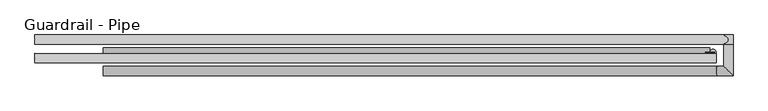
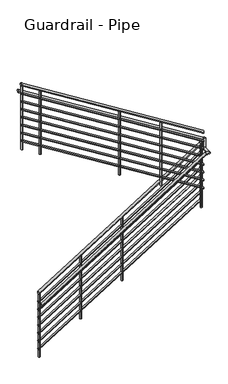
"""IFC4 building model written with IfcOpenShell, lengths in millimetres: railing geometry, Guardrail - Pipe."""

from ifc_helpers import new_model, si_unit, point, frame, frame_2d, origin, place, context, project, spatial, circle_curve, ellipse_curve, trimmed, segment, composite_curve, outline, extrude, faceted_brep, source, transform, mapped, element, save
from ifc_brep_helpers import plane_surface, cylinder_surface, advanced_brep


def guardrail_pipe_d6e5a110(model_context):
    return source(origin(), model_context, "Body", "SolidModel", [
        advanced_brep(
        [(-2631.8939612, 10554.0699505, -2439.0768639), (-2631.8939612, 10515.9699505, -2439.0768639), (-142.6939612, 10554.0699505, -887.367773), (-142.6939612, 10515.9699505, -887.367773)],
        [
            (0, 1, ellipse_curve(frame((-2631.8939612, 10535.0199505, -2439.0768639), z_axis=(-1.0, 0.0, 0.0), x_axis=(0.0, 0.0, -1.0)), 22.4482925, 19.05)),
            (1, 0, ellipse_curve(frame((-2631.8939612, 10535.0199505, -2439.0768639), z_axis=(-1.0, 0.0, 0.0), x_axis=(0.0, 0.0, -1.0)), 22.4482925, 19.05)),
            (2, 3, ellipse_curve(frame((-142.6939612, 10535.0199505, -887.367773), z_axis=(1.0, 0.0, 0.0), x_axis=(0.0, 0.0, -1.0)), 22.4482925, 19.05)),
            (3, 2, ellipse_curve(frame((-142.6939612, 10535.0199505, -887.367773), z_axis=(1.0, 0.0, 0.0), x_axis=(0.0, 0.0, -1.0)), 22.4482925, 19.05)),
            (0, 2),
            (3, 1),
        ],
        [
            plane_surface(frame((-2631.8939612, 10535.0199505, -2416.6285714), z_axis=(-1.0, 0.0, 0.0), x_axis=(0.0, 1.0, 0.0))),
            plane_surface(frame((-142.6939612, 10535.0199505, -864.9194805), z_axis=(1.0, 0.0, 0.0), x_axis=(0.0, 1.0, 0.0))),
            cylinder_surface(frame((-2621.8163602, 10535.0199505, -2432.794723), z_axis=(-0.8486168825713737, 0.0, -0.5290079267977406), x_axis=(0.0, -1.0, 0.0)), 19.05),
        ],
        [
            (0, [[1, 2]]),
            (1, [[3, 4]]),
            (2, [[-1, 5, -4, 6]]),
            (2, [[-2, -6, -3, -5]]),
        ],
    ),
        advanced_brep(
        [(-161.7439612, 10535.0199505, -868.1357143), (-123.6439612, 10535.0199505, -868.1357143), (-161.7439612, 10536.659643, -868.1357143), (-123.6439612, 10536.659643, -868.1357143)],
        [
            (0, 1, circle_curve(frame((-142.6939612, 10535.0199505, -868.1357143), z_axis=(0.0, -1.0, 0.0), x_axis=(1.0, 0.0, 0.0)), 19.05)),
            (1, 0, circle_curve(frame((-142.6939612, 10535.0199505, -868.1357143), z_axis=(0.0, -1.0, 0.0), x_axis=(1.0, 0.0, 0.0)), 19.05)),
            (2, 3, circle_curve(frame((-142.6939612, 10536.659643, -868.1357143), z_axis=(0.0, 1.0, 0.0), x_axis=(1.0, 0.0, 0.0)), 19.05)),
            (3, 2, circle_curve(frame((-142.6939612, 10536.659643, -868.1357143), z_axis=(0.0, 1.0, 0.0), x_axis=(1.0, 0.0, 0.0)), 19.05)),
            (0, 2),
            (3, 1),
        ],
        [
            plane_surface(frame((-142.6939612, 10535.0199505, -849.0857143), z_axis=(0.0, -1.0, 0.0), x_axis=(0.0, 0.0, 1.0))),
            plane_surface(frame((-142.6939612, 10536.659643, -849.0857143), z_axis=(0.0, 1.0, 0.0), x_axis=(0.0, 0.0, 1.0))),
            cylinder_surface(frame((-142.6939612, 10535.0199505, -868.1357143), z_axis=(0.0, -1.0, 0.0), x_axis=(1.0, 0.0, 0.0)), 19.05),
        ],
        [
            (0, [[1, 2]]),
            (1, [[3, 4]]),
            (2, [[-1, 5, -4, 6]]),
            (2, [[-2, -6, -3, -5]]),
        ],
    ),
        advanced_brep(
        [(-117.2939612, 10492.209643, -697.3625782), (-117.2939612, 10530.309643, -697.3625782), (-2911.2939612, 10492.209643, 1044.3517075), (-2911.2939612, 10530.309643, 1044.3517075)],
        [
            (0, 1, ellipse_curve(frame((-117.2939612, 10511.259643, -697.3625782), z_axis=(1.0, 0.0, 0.0), x_axis=(0.0, 0.0, -1.0)), 22.4482925, 19.05)),
            (1, 0, ellipse_curve(frame((-117.2939612, 10511.259643, -697.3625782), z_axis=(1.0, 0.0, 0.0), x_axis=(0.0, 0.0, -1.0)), 22.4482925, 19.05)),
            (2, 3, ellipse_curve(frame((-2911.2939612, 10511.259643, 1044.3517075), z_axis=(-1.0, 0.0, 0.0), x_axis=(0.0, 0.0, -1.0)), 22.4482925, 19.05)),
            (3, 2, ellipse_curve(frame((-2911.2939612, 10511.259643, 1044.3517075), z_axis=(-1.0, 0.0, 0.0), x_axis=(0.0, 0.0, -1.0)), 22.4482925, 19.05)),
            (0, 2),
            (3, 1),
        ],
        [
            plane_surface(frame((-117.2939612, 10511.259643, -674.9142857), z_axis=(1.0, 0.0, 0.0), x_axis=(0.0, -1.0, 0.0))),
            plane_surface(frame((-2911.2939612, 10511.259643, 1066.8), z_axis=(-1.0, 0.0, 0.0), x_axis=(0.0, -1.0, 0.0))),
            cylinder_surface(frame((-127.3715622, 10511.259643, -691.0804373), z_axis=(0.8486168825713738, 0.0, -0.5290079267977402), x_axis=(0.0, 1.0, 0.0)), 19.05),
        ],
        [
            (0, [[1, 2]]),
            (1, [[3, 4]]),
            (2, [[-1, 5, -4, 6]]),
            (2, [[-2, -6, -3, -5]]),
        ],
    ),
        advanced_brep(
        [(-2631.8939612, 10547.7199505, -2583.9940998), (-2631.8939612, 10522.3199505, -2583.9940998), (-142.6939612, 10547.7199505, -1032.2850089), (-142.6939612, 10522.3199505, -1032.2850089)],
        [
            (0, 1, ellipse_curve(frame((-2631.8939612, 10535.0199505, -2583.9940998), z_axis=(-1.0, 0.0, 0.0), x_axis=(0.0, 0.0, -1.0)), 14.9655283, 12.7)),
            (1, 0, ellipse_curve(frame((-2631.8939612, 10535.0199505, -2583.9940998), z_axis=(-1.0, 0.0, 0.0), x_axis=(0.0, 0.0, -1.0)), 14.9655283, 12.7)),
            (2, 3, ellipse_curve(frame((-142.6939612, 10535.0199505, -1032.2850089), z_axis=(1.0, 0.0, 0.0), x_axis=(0.0, 0.0, -1.0)), 14.9655283, 12.7)),
            (3, 2, ellipse_curve(frame((-142.6939612, 10535.0199505, -1032.2850089), z_axis=(1.0, 0.0, 0.0), x_axis=(0.0, 0.0, -1.0)), 14.9655283, 12.7)),
            (0, 2),
            (3, 1),
        ],
        [
            plane_surface(frame((-2631.8939612, 10535.0199505, -2569.0285714), z_axis=(-1.0, 0.0, 0.0), x_axis=(0.0, 1.0, 0.0))),
            plane_surface(frame((-142.6939612, 10535.0199505, -1017.3194805), z_axis=(1.0, 0.0, 0.0), x_axis=(0.0, 1.0, 0.0))),
            cylinder_surface(frame((-2625.1755605, 10535.0199505, -2579.8060058), z_axis=(-0.8486168825713737, 0.0, -0.5290079267977406), x_axis=(0.0, -1.0, 0.0)), 12.7),
        ],
        [
            (0, [[1, 2]]),
            (1, [[3, 4]]),
            (2, [[-1, 5, -4, 6]]),
            (2, [[-2, -6, -3, -5]]),
        ],
    ),
        advanced_brep(
        [(-155.3939612, 10535.0199505, -1014.1857143), (-129.9939612, 10535.0199505, -1014.1857143), (-155.3939612, 10536.659643, -1014.1857143), (-129.9939612, 10536.659643, -1014.1857143)],
        [
            (0, 1, circle_curve(frame((-142.6939612, 10535.0199505, -1014.1857143), z_axis=(0.0, -1.0, 0.0), x_axis=(1.0, 0.0, 0.0)), 12.7)),
            (1, 0, circle_curve(frame((-142.6939612, 10535.0199505, -1014.1857143), z_axis=(0.0, -1.0, 0.0), x_axis=(1.0, 0.0, 0.0)), 12.7)),
            (2, 3, circle_curve(frame((-142.6939612, 10536.659643, -1014.1857143), z_axis=(0.0, 1.0, 0.0), x_axis=(1.0, 0.0, 0.0)), 12.7)),
            (3, 2, circle_curve(frame((-142.6939612, 10536.659643, -1014.1857143), z_axis=(0.0, 1.0, 0.0), x_axis=(1.0, 0.0, 0.0)), 12.7)),
            (0, 2),
            (3, 1),
        ],
        [
            plane_surface(frame((-142.6939612, 10535.0199505, -1001.4857143), z_axis=(0.0, -1.0, 0.0), x_axis=(0.0, 0.0, 1.0))),
            plane_surface(frame((-142.6939612, 10536.659643, -1001.4857143), z_axis=(0.0, 1.0, 0.0), x_axis=(0.0, 0.0, 1.0))),
            cylinder_surface(frame((-142.6939612, 10535.0199505, -1014.1857143), z_axis=(0.0, -1.0, 0.0), x_axis=(1.0, 0.0, 0.0)), 12.7),
        ],
        [
            (0, [[1, 2]]),
            (1, [[3, 4]]),
            (2, [[-1, 5, -4, 6]]),
            (2, [[-2, -6, -3, -5]]),
        ],
    ),
        advanced_brep(
        [(-117.2939612, 10498.559643, -842.279814), (-117.2939612, 10523.959643, -842.279814), (-2911.2939612, 10498.559643, 899.4344717), (-2911.2939612, 10523.959643, 899.4344717)],
        [
            (0, 1, ellipse_curve(frame((-117.2939612, 10511.259643, -842.279814), z_axis=(1.0, 0.0, 0.0), x_axis=(0.0, 0.0, -1.0)), 14.9655283, 12.7)),
            (1, 0, ellipse_curve(frame((-117.2939612, 10511.259643, -842.279814), z_axis=(1.0, 0.0, 0.0), x_axis=(0.0, 0.0, -1.0)), 14.9655283, 12.7)),
            (2, 3, ellipse_curve(frame((-2911.2939612, 10511.259643, 899.4344717), z_axis=(-1.0, 0.0, 0.0), x_axis=(0.0, 0.0, -1.0)), 14.9655283, 12.7)),
            (3, 2, ellipse_curve(frame((-2911.2939612, 10511.259643, 899.4344717), z_axis=(-1.0, 0.0, 0.0), x_axis=(0.0, 0.0, -1.0)), 14.9655283, 12.7)),
            (0, 2),
            (3, 1),
        ],
        [
            plane_surface(frame((-117.2939612, 10511.259643, -827.3142857), z_axis=(1.0, 0.0, 0.0), x_axis=(0.0, -1.0, 0.0))),
            plane_surface(frame((-2911.2939612, 10511.259643, 914.4), z_axis=(-1.0, 0.0, 0.0), x_axis=(0.0, -1.0, 0.0))),
            cylinder_surface(frame((-124.0123619, 10511.259643, -838.0917201), z_axis=(0.8486168825713738, 0.0, -0.5290079267977402), x_axis=(0.0, 1.0, 0.0)), 12.7),
        ],
        [
            (0, [[1, 2]]),
            (1, [[3, 4]]),
            (2, [[-1, 5, -4, 6]]),
            (2, [[-2, -6, -3, -5]]),
        ],
    ),
        advanced_brep(
        [(-2631.8939612, 10477.8699505, -2591.4768639), (-2631.8939612, 10439.7699505, -2591.4768639), (-111.8425336, 10477.8699505, -1020.5357143), (-111.8425336, 10439.7699505, -1020.5357143), (-85.5439612, 10477.8699505, -1020.5357143), (-47.4439612, 10439.7699505, -1020.5357143), (-85.5439612, 10587.459643, -1020.5357143), (-47.4439612, 10587.459643, -1020.5357143)],
        [
            (0, 1, ellipse_curve(frame((-2631.8939612, 10458.8199505, -2591.4768639), z_axis=(-1.0, 0.0, 0.0), x_axis=(0.0, 0.0, -1.0)), 22.4482925, 19.05)),
            (1, 0, ellipse_curve(frame((-2631.8939612, 10458.8199505, -2591.4768639), z_axis=(-1.0, 0.0, 0.0), x_axis=(0.0, 0.0, -1.0)), 22.4482925, 19.05)),
            (0, 2),
            (2, 3, ellipse_curve(frame((-111.8425336, 10458.8199505, -1020.5357143), z_axis=(-0.9614096116045889, 0.0, -0.275120989228945), x_axis=(0.27512098922894457, 0.0, -0.9614096116045892)), 19.8146552, 19.05)),
            (3, 1),
            (3, 2, ellipse_curve(frame((-111.8425336, 10458.8199505, -1020.5357143), z_axis=(-0.9614096116045889, 0.0, -0.275120989228945), x_axis=(0.27512098922894457, 0.0, -0.9614096116045892)), 19.8146552, 19.05)),
            (2, 4),
            (4, 5, ellipse_curve(frame((-66.4939612, 10458.8199505, -1020.5357143), z_axis=(-0.7071067811865475, -0.7071067811865475, 0.0), x_axis=(-0.7071067811865476, 0.7071067811865474, 0.0)), 26.9407684, 19.05)),
            (5, 3),
            (5, 4, ellipse_curve(frame((-66.4939612, 10458.8199505, -1020.5357143), z_axis=(-0.7071067811865475, -0.7071067811865475, 0.0), x_axis=(-0.7071067811865476, 0.7071067811865474, 0.0)), 26.9407684, 19.05)),
            (6, 7, circle_curve(frame((-66.4939612, 10587.459643, -1020.5357143), z_axis=(0.0, 1.0, 0.0), x_axis=(1.0, 0.0, 0.0)), 19.05)),
            (7, 6, circle_curve(frame((-66.4939612, 10587.459643, -1020.5357143), z_axis=(0.0, 1.0, 0.0), x_axis=(1.0, 0.0, 0.0)), 19.05)),
            (4, 6),
            (7, 5),
        ],
        [
            plane_surface(frame((-2631.8939612, 10458.8199505, -2569.0285714), z_axis=(-1.0, 0.0, 0.0), x_axis=(0.0, 1.0, 0.0))),
            cylinder_surface(frame((-2621.8163602, 10458.8199505, -2585.194723), z_axis=(-0.8486168825713737, 0.0, -0.5290079267977406), x_axis=(0.0, -1.0, 0.0)), 19.05),
            cylinder_surface(frame((-117.2939612, 10458.8199505, -1020.5357143), z_axis=(-1.0, 0.0, 0.0), x_axis=(0.0, -1.0, 0.0)), 19.05),
            plane_surface(frame((-66.4939612, 10587.459643, -1001.4857143), z_axis=(0.0, 1.0, 0.0), x_axis=(0.0, 0.0, 1.0))),
            cylinder_surface(frame((-66.4939612, 10458.8199505, -1020.5357143), z_axis=(0.0, -1.0, 0.0), x_axis=(1.0, 0.0, 0.0)), 19.05),
        ],
        [
            (0, [[1, 2]]),
            (1, [[-1, 3, 4, 5]]),
            (1, [[-2, -5, 6, -3]]),
            (2, [[-4, 7, 8, 9]]),
            (2, [[-6, -9, 10, -7]]),
            (3, [[11, 12]]),
            (4, [[-8, 13, -12, 14]]),
            (4, [[-10, -14, -11, -13]]),
        ],
    ),
        faceted_brep([(-85.5439612, 10606.509643, -1039.5857143), (-47.4439612, 10606.509643, -1039.5857143), (-47.4439612, 10568.409643, -1039.5857143), (-85.5439612, 10568.409643, -1039.5857143), (-85.5439612, 10606.509643, -858.9818182), (-85.5439612, 10568.409643, -858.9818182), (-47.4439612, 10568.409643, -858.9818182), (-47.4439612, 10606.509643, -858.9818182)], [[[0, 1, 2, 3]], [[4, 5, 6, 7]], [[1, 0, 4, 7]], [[2, 1, 7, 6]], [[3, 2, 6, 5]], [[0, 3, 5, 4]]]),
        advanced_brep(
        [(-66.4939612, 10568.409643, -881.4301107), (-66.4939612, 10606.509643, -881.4301107), (-2911.2939612, 10568.409643, 891.9517075), (-2911.2939612, 10606.509643, 891.9517075)],
        [
            (0, 1, ellipse_curve(frame((-66.4939612, 10587.459643, -881.4301107), z_axis=(1.0, 0.0, 0.0), x_axis=(0.0, 0.0, -1.0)), 22.4482925, 19.05)),
            (1, 0, ellipse_curve(frame((-66.4939612, 10587.459643, -881.4301107), z_axis=(1.0, 0.0, 0.0), x_axis=(0.0, 0.0, -1.0)), 22.4482925, 19.05)),
            (2, 3, ellipse_curve(frame((-2911.2939612, 10587.459643, 891.9517075), z_axis=(-1.0, 0.0, 0.0), x_axis=(0.0, 0.0, -1.0)), 22.4482925, 19.05)),
            (3, 2, ellipse_curve(frame((-2911.2939612, 10587.459643, 891.9517075), z_axis=(-1.0, 0.0, 0.0), x_axis=(0.0, 0.0, -1.0)), 22.4482925, 19.05)),
            (0, 2),
            (3, 1),
        ],
        [
            plane_surface(frame((-66.4939612, 10587.459643, -858.9818182), z_axis=(1.0, 0.0, 0.0), x_axis=(0.0, -1.0, 0.0))),
            plane_surface(frame((-2911.2939612, 10587.459643, 914.4), z_axis=(-1.0, 0.0, 0.0), x_axis=(0.0, -1.0, 0.0))),
            cylinder_surface(frame((-76.5715622, 10587.459643, -875.1479698), z_axis=(0.8486168825713738, 0.0, -0.5290079267977402), x_axis=(0.0, 1.0, 0.0)), 19.05),
        ],
        [
            (0, [[1, 2]]),
            (1, [[3, 4]]),
            (2, [[-1, 5, -4, 6]]),
            (2, [[-2, -6, -3, -5]]),
        ],
    ),
        advanced_brep(
        [(-2631.8939612, 10547.7199505, -2710.9940998), (-2631.8939612, 10522.3199505, -2710.9940998), (-142.6939612, 10547.7199505, -1159.2850089), (-142.6939612, 10522.3199505, -1159.2850089)],
        [
            (0, 1, ellipse_curve(frame((-2631.8939612, 10535.0199505, -2710.9940998), z_axis=(-1.0, 0.0, 0.0), x_axis=(0.0, 0.0, -1.0)), 14.9655283, 12.7)),
            (1, 0, ellipse_curve(frame((-2631.8939612, 10535.0199505, -2710.9940998), z_axis=(-1.0, 0.0, 0.0), x_axis=(0.0, 0.0, -1.0)), 14.9655283, 12.7)),
            (2, 3, ellipse_curve(frame((-142.6939612, 10535.0199505, -1159.2850089), z_axis=(1.0, 0.0, 0.0), x_axis=(0.0, 0.0, -1.0)), 14.9655283, 12.7)),
            (3, 2, ellipse_curve(frame((-142.6939612, 10535.0199505, -1159.2850089), z_axis=(1.0, 0.0, 0.0), x_axis=(0.0, 0.0, -1.0)), 14.9655283, 12.7)),
            (0, 2),
            (3, 1),
        ],
        [
            plane_surface(frame((-2631.8939612, 10535.0199505, -2696.0285714), z_axis=(-1.0, 0.0, 0.0), x_axis=(0.0, 1.0, 0.0))),
            plane_surface(frame((-142.6939612, 10535.0199505, -1144.3194805), z_axis=(1.0, 0.0, 0.0), x_axis=(0.0, 1.0, 0.0))),
            cylinder_surface(frame((-2625.1755605, 10535.0199505, -2706.8060058), z_axis=(-0.8486168825713737, 0.0, -0.5290079267977406), x_axis=(0.0, -1.0, 0.0)), 12.7),
        ],
        [
            (0, [[1, 2]]),
            (1, [[3, 4]]),
            (2, [[-1, 5, -4, 6]]),
            (2, [[-2, -6, -3, -5]]),
        ],
    ),
        advanced_brep(
        [(-155.3939612, 10535.0199505, -1141.1857143), (-129.9939612, 10535.0199505, -1141.1857143), (-155.3939612, 10536.659643, -1141.1857143), (-129.9939612, 10536.659643, -1141.1857143)],
        [
            (0, 1, circle_curve(frame((-142.6939612, 10535.0199505, -1141.1857143), z_axis=(0.0, -1.0, 0.0), x_axis=(1.0, 0.0, 0.0)), 12.7)),
            (1, 0, circle_curve(frame((-142.6939612, 10535.0199505, -1141.1857143), z_axis=(0.0, -1.0, 0.0), x_axis=(1.0, 0.0, 0.0)), 12.7)),
            (2, 3, circle_curve(frame((-142.6939612, 10536.659643, -1141.1857143), z_axis=(0.0, 1.0, 0.0), x_axis=(1.0, 0.0, 0.0)), 12.7)),
            (3, 2, circle_curve(frame((-142.6939612, 10536.659643, -1141.1857143), z_axis=(0.0, 1.0, 0.0), x_axis=(1.0, 0.0, 0.0)), 12.7)),
            (0, 2),
            (3, 1),
        ],
        [
            plane_surface(frame((-142.6939612, 10535.0199505, -1128.4857143), z_axis=(0.0, -1.0, 0.0), x_axis=(0.0, 0.0, 1.0))),
            plane_surface(frame((-142.6939612, 10536.659643, -1128.4857143), z_axis=(0.0, 1.0, 0.0), x_axis=(0.0, 0.0, 1.0))),
            cylinder_surface(frame((-142.6939612, 10535.0199505, -1141.1857143), z_axis=(0.0, -1.0, 0.0), x_axis=(1.0, 0.0, 0.0)), 12.7),
        ],
        [
            (0, [[1, 2]]),
            (1, [[3, 4]]),
            (2, [[-1, 5, -4, 6]]),
            (2, [[-2, -6, -3, -5]]),
        ],
    ),
        advanced_brep(
        [(-117.2939612, 10498.559643, -969.279814), (-117.2939612, 10523.959643, -969.279814), (-2911.2939612, 10498.559643, 772.4344717), (-2911.2939612, 10523.959643, 772.4344717)],
        [
            (0, 1, ellipse_curve(frame((-117.2939612, 10511.259643, -969.279814), z_axis=(1.0, 0.0, 0.0), x_axis=(0.0, 0.0, -1.0)), 14.9655283, 12.7)),
            (1, 0, ellipse_curve(frame((-117.2939612, 10511.259643, -969.279814), z_axis=(1.0, 0.0, 0.0), x_axis=(0.0, 0.0, -1.0)), 14.9655283, 12.7)),
            (2, 3, ellipse_curve(frame((-2911.2939612, 10511.259643, 772.4344717), z_axis=(-1.0, 0.0, 0.0), x_axis=(0.0, 0.0, -1.0)), 14.9655283, 12.7)),
            (3, 2, ellipse_curve(frame((-2911.2939612, 10511.259643, 772.4344717), z_axis=(-1.0, 0.0, 0.0), x_axis=(0.0, 0.0, -1.0)), 14.9655283, 12.7)),
            (0, 2),
            (3, 1),
        ],
        [
            plane_surface(frame((-117.2939612, 10511.259643, -954.3142857), z_axis=(1.0, 0.0, 0.0), x_axis=(0.0, -1.0, 0.0))),
            plane_surface(frame((-2911.2939612, 10511.259643, 787.4), z_axis=(-1.0, 0.0, 0.0), x_axis=(0.0, -1.0, 0.0))),
            cylinder_surface(frame((-124.0123619, 10511.259643, -965.0917201), z_axis=(0.8486168825713738, 0.0, -0.5290079267977402), x_axis=(0.0, 1.0, 0.0)), 12.7),
        ],
        [
            (0, [[1, 2]]),
            (1, [[3, 4]]),
            (2, [[-1, 5, -4, 6]]),
            (2, [[-2, -6, -3, -5]]),
        ],
    ),
        advanced_brep(
        [(-2631.8939612, 10547.7199505, -2837.9940998), (-2631.8939612, 10522.3199505, -2837.9940998), (-142.6939612, 10547.7199505, -1286.2850089), (-142.6939612, 10522.3199505, -1286.2850089)],
        [
            (0, 1, ellipse_curve(frame((-2631.8939612, 10535.0199505, -2837.9940998), z_axis=(-1.0, 0.0, 0.0), x_axis=(0.0, 0.0, -1.0)), 14.9655283, 12.7)),
            (1, 0, ellipse_curve(frame((-2631.8939612, 10535.0199505, -2837.9940998), z_axis=(-1.0, 0.0, 0.0), x_axis=(0.0, 0.0, -1.0)), 14.9655283, 12.7)),
            (2, 3, ellipse_curve(frame((-142.6939612, 10535.0199505, -1286.2850089), z_axis=(1.0, 0.0, 0.0), x_axis=(0.0, 0.0, -1.0)), 14.9655283, 12.7)),
            (3, 2, ellipse_curve(frame((-142.6939612, 10535.0199505, -1286.2850089), z_axis=(1.0, 0.0, 0.0), x_axis=(0.0, 0.0, -1.0)), 14.9655283, 12.7)),
            (0, 2),
            (3, 1),
        ],
        [
            plane_surface(frame((-2631.8939612, 10535.0199505, -2823.0285714), z_axis=(-1.0, 0.0, 0.0), x_axis=(0.0, 1.0, 0.0))),
            plane_surface(frame((-142.6939612, 10535.0199505, -1271.3194805), z_axis=(1.0, 0.0, 0.0), x_axis=(0.0, 1.0, 0.0))),
            cylinder_surface(frame((-2625.1755605, 10535.0199505, -2833.8060058), z_axis=(-0.8486168825713737, 0.0, -0.5290079267977406), x_axis=(0.0, -1.0, 0.0)), 12.7),
        ],
        [
            (0, [[1, 2]]),
            (1, [[3, 4]]),
            (2, [[-1, 5, -4, 6]]),
            (2, [[-2, -6, -3, -5]]),
        ],
    ),
        advanced_brep(
        [(-155.3939612, 10535.0199505, -1268.1857143), (-129.9939612, 10535.0199505, -1268.1857143), (-155.3939612, 10536.659643, -1268.1857143), (-129.9939612, 10536.659643, -1268.1857143)],
        [
            (0, 1, circle_curve(frame((-142.6939612, 10535.0199505, -1268.1857143), z_axis=(0.0, -1.0, 0.0), x_axis=(1.0, 0.0, 0.0)), 12.7)),
            (1, 0, circle_curve(frame((-142.6939612, 10535.0199505, -1268.1857143), z_axis=(0.0, -1.0, 0.0), x_axis=(1.0, 0.0, 0.0)), 12.7)),
            (2, 3, circle_curve(frame((-142.6939612, 10536.659643, -1268.1857143), z_axis=(0.0, 1.0, 0.0), x_axis=(1.0, 0.0, 0.0)), 12.7)),
            (3, 2, circle_curve(frame((-142.6939612, 10536.659643, -1268.1857143), z_axis=(0.0, 1.0, 0.0), x_axis=(1.0, 0.0, 0.0)), 12.7)),
            (0, 2),
            (3, 1),
        ],
        [
            plane_surface(frame((-142.6939612, 10535.0199505, -1255.4857143), z_axis=(0.0, -1.0, 0.0), x_axis=(0.0, 0.0, 1.0))),
            plane_surface(frame((-142.6939612, 10536.659643, -1255.4857143), z_axis=(0.0, 1.0, 0.0), x_axis=(0.0, 0.0, 1.0))),
            cylinder_surface(frame((-142.6939612, 10535.0199505, -1268.1857143), z_axis=(0.0, -1.0, 0.0), x_axis=(1.0, 0.0, 0.0)), 12.7),
        ],
        [
            (0, [[1, 2]]),
            (1, [[3, 4]]),
            (2, [[-1, 5, -4, 6]]),
            (2, [[-2, -6, -3, -5]]),
        ],
    ),
        advanced_brep(
        [(-117.2939612, 10498.559643, -1096.279814), (-117.2939612, 10523.959643, -1096.279814), (-2911.2939612, 10498.559643, 645.4344717), (-2911.2939612, 10523.959643, 645.4344717)],
        [
            (0, 1, ellipse_curve(frame((-117.2939612, 10511.259643, -1096.279814), z_axis=(1.0, 0.0, 0.0), x_axis=(0.0, 0.0, -1.0)), 14.9655283, 12.7)),
            (1, 0, ellipse_curve(frame((-117.2939612, 10511.259643, -1096.279814), z_axis=(1.0, 0.0, 0.0), x_axis=(0.0, 0.0, -1.0)), 14.9655283, 12.7)),
            (2, 3, ellipse_curve(frame((-2911.2939612, 10511.259643, 645.4344717), z_axis=(-1.0, 0.0, 0.0), x_axis=(0.0, 0.0, -1.0)), 14.9655283, 12.7)),
            (3, 2, ellipse_curve(frame((-2911.2939612, 10511.259643, 645.4344717), z_axis=(-1.0, 0.0, 0.0), x_axis=(0.0, 0.0, -1.0)), 14.9655283, 12.7)),
            (0, 2),
            (3, 1),
        ],
        [
            plane_surface(frame((-117.2939612, 10511.259643, -1081.3142857), z_axis=(1.0, 0.0, 0.0), x_axis=(0.0, -1.0, 0.0))),
            plane_surface(frame((-2911.2939612, 10511.259643, 660.4), z_axis=(-1.0, 0.0, 0.0), x_axis=(0.0, -1.0, 0.0))),
            cylinder_surface(frame((-124.0123619, 10511.259643, -1092.0917201), z_axis=(0.8486168825713738, 0.0, -0.5290079267977402), x_axis=(0.0, 1.0, 0.0)), 12.7),
        ],
        [
            (0, [[1, 2]]),
            (1, [[3, 4]]),
            (2, [[-1, 5, -4, 6]]),
            (2, [[-2, -6, -3, -5]]),
        ],
    ),
        advanced_brep(
        [(-2631.8939612, 10547.7199505, -2964.9940998), (-2631.8939612, 10522.3199505, -2964.9940998), (-142.6939612, 10547.7199505, -1413.2850089), (-142.6939612, 10522.3199505, -1413.2850089)],
        [
            (0, 1, ellipse_curve(frame((-2631.8939612, 10535.0199505, -2964.9940998), z_axis=(-1.0, 0.0, 0.0), x_axis=(0.0, 0.0, -1.0)), 14.9655283, 12.7)),
            (1, 0, ellipse_curve(frame((-2631.8939612, 10535.0199505, -2964.9940998), z_axis=(-1.0, 0.0, 0.0), x_axis=(0.0, 0.0, -1.0)), 14.9655283, 12.7)),
            (2, 3, ellipse_curve(frame((-142.6939612, 10535.0199505, -1413.2850089), z_axis=(1.0, 0.0, 0.0), x_axis=(0.0, 0.0, -1.0)), 14.9655283, 12.7)),
            (3, 2, ellipse_curve(frame((-142.6939612, 10535.0199505, -1413.2850089), z_axis=(1.0, 0.0, 0.0), x_axis=(0.0, 0.0, -1.0)), 14.9655283, 12.7)),
            (0, 2),
            (3, 1),
        ],
        [
            plane_surface(frame((-2631.8939612, 10535.0199505, -2950.0285714), z_axis=(-1.0, 0.0, 0.0), x_axis=(0.0, 1.0, 0.0))),
            plane_surface(frame((-142.6939612, 10535.0199505, -1398.3194805), z_axis=(1.0, 0.0, 0.0), x_axis=(0.0, 1.0, 0.0))),
            cylinder_surface(frame((-2625.1755605, 10535.0199505, -2960.8060058), z_axis=(-0.8486168825713737, 0.0, -0.5290079267977406), x_axis=(0.0, -1.0, 0.0)), 12.7),
        ],
        [
            (0, [[1, 2]]),
            (1, [[3, 4]]),
            (2, [[-1, 5, -4, 6]]),
            (2, [[-2, -6, -3, -5]]),
        ],
    ),
        advanced_brep(
        [(-155.3939612, 10535.0199505, -1395.1857143), (-129.9939612, 10535.0199505, -1395.1857143), (-155.3939612, 10536.659643, -1395.1857143), (-129.9939612, 10536.659643, -1395.1857143)],
        [
            (0, 1, circle_curve(frame((-142.6939612, 10535.0199505, -1395.1857143), z_axis=(0.0, -1.0, 0.0), x_axis=(1.0, 0.0, 0.0)), 12.7)),
            (1, 0, circle_curve(frame((-142.6939612, 10535.0199505, -1395.1857143), z_axis=(0.0, -1.0, 0.0), x_axis=(1.0, 0.0, 0.0)), 12.7)),
            (2, 3, circle_curve(frame((-142.6939612, 10536.659643, -1395.1857143), z_axis=(0.0, 1.0, 0.0), x_axis=(1.0, 0.0, 0.0)), 12.7)),
            (3, 2, circle_curve(frame((-142.6939612, 10536.659643, -1395.1857143), z_axis=(0.0, 1.0, 0.0), x_axis=(1.0, 0.0, 0.0)), 12.7)),
            (0, 2),
            (3, 1),
        ],
        [
            plane_surface(frame((-142.6939612, 10535.0199505, -1382.4857143), z_axis=(0.0, -1.0, 0.0), x_axis=(0.0, 0.0, 1.0))),
            plane_surface(frame((-142.6939612, 10536.659643, -1382.4857143), z_axis=(0.0, 1.0, 0.0), x_axis=(0.0, 0.0, 1.0))),
            cylinder_surface(frame((-142.6939612, 10535.0199505, -1395.1857143), z_axis=(0.0, -1.0, 0.0), x_axis=(1.0, 0.0, 0.0)), 12.7),
        ],
        [
            (0, [[1, 2]]),
            (1, [[3, 4]]),
            (2, [[-1, 5, -4, 6]]),
            (2, [[-2, -6, -3, -5]]),
        ],
    ),
        advanced_brep(
        [(-117.2939612, 10498.559643, -1223.279814), (-117.2939612, 10523.959643, -1223.279814), (-2911.2939612, 10498.559643, 518.4344717), (-2911.2939612, 10523.959643, 518.4344717)],
        [
            (0, 1, ellipse_curve(frame((-117.2939612, 10511.259643, -1223.279814), z_axis=(1.0, 0.0, 0.0), x_axis=(0.0, 0.0, -1.0)), 14.9655283, 12.7)),
            (1, 0, ellipse_curve(frame((-117.2939612, 10511.259643, -1223.279814), z_axis=(1.0, 0.0, 0.0), x_axis=(0.0, 0.0, -1.0)), 14.9655283, 12.7)),
            (2, 3, ellipse_curve(frame((-2911.2939612, 10511.259643, 518.4344717), z_axis=(-1.0, 0.0, 0.0), x_axis=(0.0, 0.0, -1.0)), 14.9655283, 12.7)),
            (3, 2, ellipse_curve(frame((-2911.2939612, 10511.259643, 518.4344717), z_axis=(-1.0, 0.0, 0.0), x_axis=(0.0, 0.0, -1.0)), 14.9655283, 12.7)),
            (0, 2),
            (3, 1),
        ],
        [
            plane_surface(frame((-117.2939612, 10511.259643, -1208.3142857), z_axis=(1.0, 0.0, 0.0), x_axis=(0.0, -1.0, 0.0))),
            plane_surface(frame((-2911.2939612, 10511.259643, 533.4), z_axis=(-1.0, 0.0, 0.0), x_axis=(0.0, -1.0, 0.0))),
            cylinder_surface(frame((-124.0123619, 10511.259643, -1219.0917201), z_axis=(0.8486168825713738, 0.0, -0.5290079267977402), x_axis=(0.0, 1.0, 0.0)), 12.7),
        ],
        [
            (0, [[1, 2]]),
            (1, [[3, 4]]),
            (2, [[-1, 5, -4, 6]]),
            (2, [[-2, -6, -3, -5]]),
        ],
    ),
        advanced_brep(
        [(-2631.8939612, 10547.7199505, -3091.9940998), (-2631.8939612, 10522.3199505, -3091.9940998), (-142.6939612, 10547.7199505, -1540.2850089), (-142.6939612, 10522.3199505, -1540.2850089)],
        [
            (0, 1, ellipse_curve(frame((-2631.8939612, 10535.0199505, -3091.9940998), z_axis=(-1.0, 0.0, 0.0), x_axis=(0.0, 0.0, -1.0)), 14.9655283, 12.7)),
            (1, 0, ellipse_curve(frame((-2631.8939612, 10535.0199505, -3091.9940998), z_axis=(-1.0, 0.0, 0.0), x_axis=(0.0, 0.0, -1.0)), 14.9655283, 12.7)),
            (2, 3, ellipse_curve(frame((-142.6939612, 10535.0199505, -1540.2850089), z_axis=(1.0, 0.0, 0.0), x_axis=(0.0, 0.0, -1.0)), 14.9655283, 12.7)),
            (3, 2, ellipse_curve(frame((-142.6939612, 10535.0199505, -1540.2850089), z_axis=(1.0, 0.0, 0.0), x_axis=(0.0, 0.0, -1.0)), 14.9655283, 12.7)),
            (0, 2),
            (3, 1),
        ],
        [
            plane_surface(frame((-2631.8939612, 10535.0199505, -3077.0285714), z_axis=(-1.0, 0.0, 0.0), x_axis=(0.0, 1.0, 0.0))),
            plane_surface(frame((-142.6939612, 10535.0199505, -1525.3194805), z_axis=(1.0, 0.0, 0.0), x_axis=(0.0, 1.0, 0.0))),
            cylinder_surface(frame((-2625.1755605, 10535.0199505, -3087.8060058), z_axis=(-0.8486168825713737, 0.0, -0.5290079267977406), x_axis=(0.0, -1.0, 0.0)), 12.7),
        ],
        [
            (0, [[1, 2]]),
            (1, [[3, 4]]),
            (2, [[-1, 5, -4, 6]]),
            (2, [[-2, -6, -3, -5]]),
        ],
    ),
        advanced_brep(
        [(-155.3939612, 10535.0199505, -1522.1857143), (-129.9939612, 10535.0199505, -1522.1857143), (-155.3939612, 10536.659643, -1522.1857143), (-129.9939612, 10536.659643, -1522.1857143)],
        [
            (0, 1, circle_curve(frame((-142.6939612, 10535.0199505, -1522.1857143), z_axis=(0.0, -1.0, 0.0), x_axis=(1.0, 0.0, 0.0)), 12.7)),
            (1, 0, circle_curve(frame((-142.6939612, 10535.0199505, -1522.1857143), z_axis=(0.0, -1.0, 0.0), x_axis=(1.0, 0.0, 0.0)), 12.7)),
            (2, 3, circle_curve(frame((-142.6939612, 10536.659643, -1522.1857143), z_axis=(0.0, 1.0, 0.0), x_axis=(1.0, 0.0, 0.0)), 12.7)),
            (3, 2, circle_curve(frame((-142.6939612, 10536.659643, -1522.1857143), z_axis=(0.0, 1.0, 0.0), x_axis=(1.0, 0.0, 0.0)), 12.7)),
            (0, 2),
            (3, 1),
        ],
        [
            plane_surface(frame((-142.6939612, 10535.0199505, -1509.4857143), z_axis=(0.0, -1.0, 0.0), x_axis=(0.0, 0.0, 1.0))),
            plane_surface(frame((-142.6939612, 10536.659643, -1509.4857143), z_axis=(0.0, 1.0, 0.0), x_axis=(0.0, 0.0, 1.0))),
            cylinder_surface(frame((-142.6939612, 10535.0199505, -1522.1857143), z_axis=(0.0, -1.0, 0.0), x_axis=(1.0, 0.0, 0.0)), 12.7),
        ],
        [
            (0, [[1, 2]]),
            (1, [[3, 4]]),
            (2, [[-1, 5, -4, 6]]),
            (2, [[-2, -6, -3, -5]]),
        ],
    ),
        advanced_brep(
        [(-117.2939612, 10498.559643, -1350.279814), (-117.2939612, 10523.959643, -1350.279814), (-2911.2939612, 10498.559643, 391.4344717), (-2911.2939612, 10523.959643, 391.4344717)],
        [
            (0, 1, ellipse_curve(frame((-117.2939612, 10511.259643, -1350.279814), z_axis=(1.0, 0.0, 0.0), x_axis=(0.0, 0.0, -1.0)), 14.9655283, 12.7)),
            (1, 0, ellipse_curve(frame((-117.2939612, 10511.259643, -1350.279814), z_axis=(1.0, 0.0, 0.0), x_axis=(0.0, 0.0, -1.0)), 14.9655283, 12.7)),
            (2, 3, ellipse_curve(frame((-2911.2939612, 10511.259643, 391.4344717), z_axis=(-1.0, 0.0, 0.0), x_axis=(0.0, 0.0, -1.0)), 14.9655283, 12.7)),
            (3, 2, ellipse_curve(frame((-2911.2939612, 10511.259643, 391.4344717), z_axis=(-1.0, 0.0, 0.0), x_axis=(0.0, 0.0, -1.0)), 14.9655283, 12.7)),
            (0, 2),
            (3, 1),
        ],
        [
            plane_surface(frame((-117.2939612, 10511.259643, -1335.3142857), z_axis=(1.0, 0.0, 0.0), x_axis=(0.0, -1.0, 0.0))),
            plane_surface(frame((-2911.2939612, 10511.259643, 406.4), z_axis=(-1.0, 0.0, 0.0), x_axis=(0.0, -1.0, 0.0))),
            cylinder_surface(frame((-124.0123619, 10511.259643, -1346.0917201), z_axis=(0.8486168825713738, 0.0, -0.5290079267977402), x_axis=(0.0, 1.0, 0.0)), 12.7),
        ],
        [
            (0, [[1, 2]]),
            (1, [[3, 4]]),
            (2, [[-1, 5, -4, 6]]),
            (2, [[-2, -6, -3, -5]]),
        ],
    ),
        advanced_brep(
        [(-2631.8939612, 10547.7199505, -3218.9940998), (-2631.8939612, 10522.3199505, -3218.9940998), (-142.6939612, 10547.7199505, -1667.2850089), (-142.6939612, 10522.3199505, -1667.2850089)],
        [
            (0, 1, ellipse_curve(frame((-2631.8939612, 10535.0199505, -3218.9940998), z_axis=(-1.0, 0.0, 0.0), x_axis=(0.0, 0.0, -1.0)), 14.9655283, 12.7)),
            (1, 0, ellipse_curve(frame((-2631.8939612, 10535.0199505, -3218.9940998), z_axis=(-1.0, 0.0, 0.0), x_axis=(0.0, 0.0, -1.0)), 14.9655283, 12.7)),
            (2, 3, ellipse_curve(frame((-142.6939612, 10535.0199505, -1667.2850089), z_axis=(1.0, 0.0, 0.0), x_axis=(0.0, 0.0, -1.0)), 14.9655283, 12.7)),
            (3, 2, ellipse_curve(frame((-142.6939612, 10535.0199505, -1667.2850089), z_axis=(1.0, 0.0, 0.0), x_axis=(0.0, 0.0, -1.0)), 14.9655283, 12.7)),
            (0, 2),
            (3, 1),
        ],
        [
            plane_surface(frame((-2631.8939612, 10535.0199505, -3204.0285714), z_axis=(-1.0, 0.0, 0.0), x_axis=(0.0, 1.0, 0.0))),
            plane_surface(frame((-142.6939612, 10535.0199505, -1652.3194805), z_axis=(1.0, 0.0, 0.0), x_axis=(0.0, 1.0, 0.0))),
            cylinder_surface(frame((-2625.1755605, 10535.0199505, -3214.8060058), z_axis=(-0.8486168825713737, 0.0, -0.5290079267977406), x_axis=(0.0, -1.0, 0.0)), 12.7),
        ],
        [
            (0, [[1, 2]]),
            (1, [[3, 4]]),
            (2, [[-1, 5, -4, 6]]),
            (2, [[-2, -6, -3, -5]]),
        ],
    ),
        advanced_brep(
        [(-155.3939612, 10535.0199505, -1649.1857143), (-129.9939612, 10535.0199505, -1649.1857143), (-155.3939612, 10536.659643, -1649.1857143), (-129.9939612, 10536.659643, -1649.1857143)],
        [
            (0, 1, circle_curve(frame((-142.6939612, 10535.0199505, -1649.1857143), z_axis=(0.0, -1.0, 0.0), x_axis=(1.0, 0.0, 0.0)), 12.7)),
            (1, 0, circle_curve(frame((-142.6939612, 10535.0199505, -1649.1857143), z_axis=(0.0, -1.0, 0.0), x_axis=(1.0, 0.0, 0.0)), 12.7)),
            (2, 3, circle_curve(frame((-142.6939612, 10536.659643, -1649.1857143), z_axis=(0.0, 1.0, 0.0), x_axis=(1.0, 0.0, 0.0)), 12.7)),
            (3, 2, circle_curve(frame((-142.6939612, 10536.659643, -1649.1857143), z_axis=(0.0, 1.0, 0.0), x_axis=(1.0, 0.0, 0.0)), 12.7)),
            (0, 2),
            (3, 1),
        ],
        [
            plane_surface(frame((-142.6939612, 10535.0199505, -1636.4857143), z_axis=(0.0, -1.0, 0.0), x_axis=(0.0, 0.0, 1.0))),
            plane_surface(frame((-142.6939612, 10536.659643, -1636.4857143), z_axis=(0.0, 1.0, 0.0), x_axis=(0.0, 0.0, 1.0))),
            cylinder_surface(frame((-142.6939612, 10535.0199505, -1649.1857143), z_axis=(0.0, -1.0, 0.0), x_axis=(1.0, 0.0, 0.0)), 12.7),
        ],
        [
            (0, [[1, 2]]),
            (1, [[3, 4]]),
            (2, [[-1, 5, -4, 6]]),
            (2, [[-2, -6, -3, -5]]),
        ],
    ),
        advanced_brep(
        [(-117.2939612, 10498.559643, -1477.279814), (-117.2939612, 10523.959643, -1477.279814), (-2911.2939612, 10498.559643, 264.4344717), (-2911.2939612, 10523.959643, 264.4344717)],
        [
            (0, 1, ellipse_curve(frame((-117.2939612, 10511.259643, -1477.279814), z_axis=(1.0, 0.0, 0.0), x_axis=(0.0, 0.0, -1.0)), 14.9655283, 12.7)),
            (1, 0, ellipse_curve(frame((-117.2939612, 10511.259643, -1477.279814), z_axis=(1.0, 0.0, 0.0), x_axis=(0.0, 0.0, -1.0)), 14.9655283, 12.7)),
            (2, 3, ellipse_curve(frame((-2911.2939612, 10511.259643, 264.4344717), z_axis=(-1.0, 0.0, 0.0), x_axis=(0.0, 0.0, -1.0)), 14.9655283, 12.7)),
            (3, 2, ellipse_curve(frame((-2911.2939612, 10511.259643, 264.4344717), z_axis=(-1.0, 0.0, 0.0), x_axis=(0.0, 0.0, -1.0)), 14.9655283, 12.7)),
            (0, 2),
            (3, 1),
        ],
        [
            plane_surface(frame((-117.2939612, 10511.259643, -1462.3142857), z_axis=(1.0, 0.0, 0.0), x_axis=(0.0, -1.0, 0.0))),
            plane_surface(frame((-2911.2939612, 10511.259643, 279.4), z_axis=(-1.0, 0.0, 0.0), x_axis=(0.0, -1.0, 0.0))),
            cylinder_surface(frame((-124.0123619, 10511.259643, -1473.0917201), z_axis=(0.8486168825713738, 0.0, -0.5290079267977402), x_axis=(0.0, 1.0, 0.0)), 12.7),
        ],
        [
            (0, [[1, 2]]),
            (1, [[3, 4]]),
            (2, [[-1, 5, -4, 6]]),
            (2, [[-2, -6, -3, -5]]),
        ],
    ),
        advanced_brep(
        [(-2631.8939612, 10547.7199505, -3345.9940998), (-2631.8939612, 10522.3199505, -3345.9940998), (-142.6939612, 10547.7199505, -1794.2850089), (-142.6939612, 10522.3199505, -1794.2850089)],
        [
            (0, 1, ellipse_curve(frame((-2631.8939612, 10535.0199505, -3345.9940998), z_axis=(-1.0, 0.0, 0.0), x_axis=(0.0, 0.0, -1.0)), 14.9655283, 12.7)),
            (1, 0, ellipse_curve(frame((-2631.8939612, 10535.0199505, -3345.9940998), z_axis=(-1.0, 0.0, 0.0), x_axis=(0.0, 0.0, -1.0)), 14.9655283, 12.7)),
            (2, 3, ellipse_curve(frame((-142.6939612, 10535.0199505, -1794.2850089), z_axis=(1.0, 0.0, 0.0), x_axis=(0.0, 0.0, -1.0)), 14.9655283, 12.7)),
            (3, 2, ellipse_curve(frame((-142.6939612, 10535.0199505, -1794.2850089), z_axis=(1.0, 0.0, 0.0), x_axis=(0.0, 0.0, -1.0)), 14.9655283, 12.7)),
            (0, 2),
            (3, 1),
        ],
        [
            plane_surface(frame((-2631.8939612, 10535.0199505, -3331.0285714), z_axis=(-1.0, 0.0, 0.0), x_axis=(0.0, 1.0, 0.0))),
            plane_surface(frame((-142.6939612, 10535.0199505, -1779.3194805), z_axis=(1.0, 0.0, 0.0), x_axis=(0.0, 1.0, 0.0))),
            cylinder_surface(frame((-2625.1755605, 10535.0199505, -3341.8060058), z_axis=(-0.8486168825713737, 0.0, -0.5290079267977406), x_axis=(0.0, -1.0, 0.0)), 12.7),
        ],
        [
            (0, [[1, 2]]),
            (1, [[3, 4]]),
            (2, [[-1, 5, -4, 6]]),
            (2, [[-2, -6, -3, -5]]),
        ],
    ),
        advanced_brep(
        [(-155.3939612, 10535.0199505, -1776.1857143), (-129.9939612, 10535.0199505, -1776.1857143), (-155.3939612, 10536.659643, -1776.1857143), (-129.9939612, 10536.659643, -1776.1857143)],
        [
            (0, 1, circle_curve(frame((-142.6939612, 10535.0199505, -1776.1857143), z_axis=(0.0, -1.0, 0.0), x_axis=(1.0, 0.0, 0.0)), 12.7)),
            (1, 0, circle_curve(frame((-142.6939612, 10535.0199505, -1776.1857143), z_axis=(0.0, -1.0, 0.0), x_axis=(1.0, 0.0, 0.0)), 12.7)),
            (2, 3, circle_curve(frame((-142.6939612, 10536.659643, -1776.1857143), z_axis=(0.0, 1.0, 0.0), x_axis=(1.0, 0.0, 0.0)), 12.7)),
            (3, 2, circle_curve(frame((-142.6939612, 10536.659643, -1776.1857143), z_axis=(0.0, 1.0, 0.0), x_axis=(1.0, 0.0, 0.0)), 12.7)),
            (0, 2),
            (3, 1),
        ],
        [
            plane_surface(frame((-142.6939612, 10535.0199505, -1763.4857143), z_axis=(0.0, -1.0, 0.0), x_axis=(0.0, 0.0, 1.0))),
            plane_surface(frame((-142.6939612, 10536.659643, -1763.4857143), z_axis=(0.0, 1.0, 0.0), x_axis=(0.0, 0.0, 1.0))),
            cylinder_surface(frame((-142.6939612, 10535.0199505, -1776.1857143), z_axis=(0.0, -1.0, 0.0), x_axis=(1.0, 0.0, 0.0)), 12.7),
        ],
        [
            (0, [[1, 2]]),
            (1, [[3, 4]]),
            (2, [[-1, 5, -4, 6]]),
            (2, [[-2, -6, -3, -5]]),
        ],
    ),
        advanced_brep(
        [(-117.2939612, 10498.559643, -1604.279814), (-117.2939612, 10523.959643, -1604.279814), (-2911.2939612, 10498.559643, 137.4344717), (-2911.2939612, 10523.959643, 137.4344717)],
        [
            (0, 1, ellipse_curve(frame((-117.2939612, 10511.259643, -1604.279814), z_axis=(1.0, 0.0, 0.0), x_axis=(0.0, 0.0, -1.0)), 14.9655283, 12.7)),
            (1, 0, ellipse_curve(frame((-117.2939612, 10511.259643, -1604.279814), z_axis=(1.0, 0.0, 0.0), x_axis=(0.0, 0.0, -1.0)), 14.9655283, 12.7)),
            (2, 3, ellipse_curve(frame((-2911.2939612, 10511.259643, 137.4344717), z_axis=(-1.0, 0.0, 0.0), x_axis=(0.0, 0.0, -1.0)), 14.9655283, 12.7)),
            (3, 2, ellipse_curve(frame((-2911.2939612, 10511.259643, 137.4344717), z_axis=(-1.0, 0.0, 0.0), x_axis=(0.0, 0.0, -1.0)), 14.9655283, 12.7)),
            (0, 2),
            (3, 1),
        ],
        [
            plane_surface(frame((-117.2939612, 10511.259643, -1589.3142857), z_axis=(1.0, 0.0, 0.0), x_axis=(0.0, -1.0, 0.0))),
            plane_surface(frame((-2911.2939612, 10511.259643, 152.4), z_axis=(-1.0, 0.0, 0.0), x_axis=(0.0, -1.0, 0.0))),
            cylinder_surface(frame((-124.0123619, 10511.259643, -1600.0917201), z_axis=(0.8486168825713738, 0.0, -0.5290079267977402), x_axis=(0.0, 1.0, 0.0)), 12.7),
        ],
        [
            (0, [[1, 2]]),
            (1, [[3, 4]]),
            (2, [[-1, 5, -4, 6]]),
            (2, [[-2, -6, -3, -5]]),
        ],
    ),
        advanced_brep(
        [(-2898.9123767, 10523.959643, -7.7183903), (-2898.9123767, 10498.559643, -7.7183903), (-2898.9123767, 10498.559643, 1014.1850247), (-2898.9123767, 10523.959643, 1014.1850247)],
        [
            (0, 1, circle_curve(frame((-2898.9123767, 10511.259643, -7.7183903), z_axis=(0.0, 0.0, -1.0), x_axis=(0.0, -1.0, 0.0)), 12.7)),
            (1, 0, circle_curve(frame((-2898.9123767, 10511.259643, -7.7183903), z_axis=(0.0, 0.0, -1.0), x_axis=(0.0, -1.0, 0.0)), 12.7)),
            (1, 2),
            (2, 3, ellipse_curve(frame((-2898.9123767, 10511.259643, 1014.1850247), z_axis=(-0.5290079267977408, 0.0, -0.8486168825713734), x_axis=(-0.8486168825713732, 0.0, 0.5290079267977408)), 14.9655283, 12.7)),
            (3, 0),
            (3, 2, ellipse_curve(frame((-2898.9123767, 10511.259643, 1014.1850247), z_axis=(-0.5290079267977408, 0.0, -0.8486168825713734), x_axis=(-0.8486168825713732, 0.0, 0.5290079267977408)), 14.9655283, 12.7)),
        ],
        [
            plane_surface(frame((-2898.9123767, 10498.559643, -7.7183903), z_axis=(0.0, 0.0, -1.0), x_axis=(-1.0, 0.0, 0.0))),
            cylinder_surface(frame((-2898.9123767, 10511.259643, -7.7183903), z_axis=(0.0, 0.0, 1.0), x_axis=(0.0, -1.0, 0.0)), 12.7),
            plane_surface(frame((-2933.8373767, 10464.0338131, 1035.9564532), z_axis=(0.5290079267977408, 0.0, 0.8486168825713734), x_axis=(0.0, 1.0, 0.0))),
        ],
        [
            (0, [[1, 2]]),
            (1, [[-2, 3, 4, 5]]),
            (1, [[-1, -5, 6, -3]]),
            (2, [[-4, -6]]),
        ],
    ),
        advanced_brep(
        [(-2619.5123767, 10523.959643, -181.8898189), (-2619.5123767, 10498.559643, -181.8898189), (-2619.5123767, 10498.559643, 840.0135961), (-2619.5123767, 10523.959643, 840.0135961)],
        [
            (0, 1, circle_curve(frame((-2619.5123767, 10511.259643, -181.8898189), z_axis=(0.0, 0.0, -1.0), x_axis=(0.0, -1.0, 0.0)), 12.7)),
            (1, 0, circle_curve(frame((-2619.5123767, 10511.259643, -181.8898189), z_axis=(0.0, 0.0, -1.0), x_axis=(0.0, -1.0, 0.0)), 12.7)),
            (1, 2),
            (2, 3, ellipse_curve(frame((-2619.5123767, 10511.259643, 840.0135961), z_axis=(-0.5290079267977408, 0.0, -0.8486168825713734), x_axis=(-0.8486168825713732, 0.0, 0.5290079267977408)), 14.9655283, 12.7)),
            (3, 0),
            (3, 2, ellipse_curve(frame((-2619.5123767, 10511.259643, 840.0135961), z_axis=(-0.5290079267977408, 0.0, -0.8486168825713734), x_axis=(-0.8486168825713732, 0.0, 0.5290079267977408)), 14.9655283, 12.7)),
        ],
        [
            plane_surface(frame((-2619.5123767, 10498.559643, -181.8898189), z_axis=(0.0, 0.0, -1.0), x_axis=(-1.0, 0.0, 0.0))),
            cylinder_surface(frame((-2619.5123767, 10511.259643, -181.8898189), z_axis=(0.0, 0.0, 1.0), x_axis=(0.0, -1.0, 0.0)), 12.7),
            plane_surface(frame((-2654.4373767, 10464.0338131, 861.7850247), z_axis=(0.5290079267977408, 0.0, 0.8486168825713734), x_axis=(0.0, 1.0, 0.0))),
        ],
        [
            (0, [[1, 2]]),
            (1, [[-2, 3, 4, 5]]),
            (1, [[-1, -5, 6, -3]]),
            (2, [[-4, -6]]),
        ],
    ),
        advanced_brep(
        [(-1400.3123767, 10523.959643, -941.9105981), (-1400.3123767, 10498.559643, -941.9105981), (-1400.3123767, 10498.559643, 79.9928169), (-1400.3123767, 10523.959643, 79.9928169)],
        [
            (0, 1, circle_curve(frame((-1400.3123767, 10511.259643, -941.9105981), z_axis=(0.0, 0.0, -1.0), x_axis=(0.0, -1.0, 0.0)), 12.7)),
            (1, 0, circle_curve(frame((-1400.3123767, 10511.259643, -941.9105981), z_axis=(0.0, 0.0, -1.0), x_axis=(0.0, -1.0, 0.0)), 12.7)),
            (1, 2),
            (2, 3, ellipse_curve(frame((-1400.3123767, 10511.259643, 79.9928169), z_axis=(-0.5290079267977408, 0.0, -0.8486168825713734), x_axis=(-0.8486168825713732, 0.0, 0.5290079267977408)), 14.9655283, 12.7)),
            (3, 0),
            (3, 2, ellipse_curve(frame((-1400.3123767, 10511.259643, 79.9928169), z_axis=(-0.5290079267977408, 0.0, -0.8486168825713734), x_axis=(-0.8486168825713732, 0.0, 0.5290079267977408)), 14.9655283, 12.7)),
        ],
        [
            plane_surface(frame((-1400.3123767, 10498.559643, -941.9105981), z_axis=(0.0, 0.0, -1.0), x_axis=(-1.0, 0.0, 0.0))),
            cylinder_surface(frame((-1400.3123767, 10511.259643, -941.9105981), z_axis=(0.0, 0.0, 1.0), x_axis=(0.0, -1.0, 0.0)), 12.7),
            plane_surface(frame((-1435.2373767, 10464.0338131, 101.7642455), z_axis=(0.5290079267977408, 0.0, 0.8486168825713734), x_axis=(0.0, 1.0, 0.0))),
        ],
        [
            (0, [[1, 2]]),
            (1, [[-2, 3, 4, 5]]),
            (1, [[-1, -5, 6, -3]]),
            (2, [[-4, -6]]),
        ],
    ),
        advanced_brep(
        [(-764.9939612, 10523.959643, -1337.9532468), (-764.9939612, 10498.559643, -1337.9532468), (-764.9939612, 10498.559643, -316.0498318), (-764.9939612, 10523.959643, -316.0498318)],
        [
            (0, 1, circle_curve(frame((-764.9939612, 10511.259643, -1337.9532468), z_axis=(0.0, 0.0, -1.0), x_axis=(0.0, -1.0, 0.0)), 12.7)),
            (1, 0, circle_curve(frame((-764.9939612, 10511.259643, -1337.9532468), z_axis=(0.0, 0.0, -1.0), x_axis=(0.0, -1.0, 0.0)), 12.7)),
            (1, 2),
            (2, 3, ellipse_curve(frame((-764.9939612, 10511.259643, -316.0498318), z_axis=(-0.5290079267977408, 0.0, -0.8486168825713734), x_axis=(-0.8486168825713732, 0.0, 0.5290079267977408)), 14.9655283, 12.7)),
            (3, 0),
            (3, 2, ellipse_curve(frame((-764.9939612, 10511.259643, -316.0498318), z_axis=(-0.5290079267977408, 0.0, -0.8486168825713734), x_axis=(-0.8486168825713732, 0.0, 0.5290079267977408)), 14.9655283, 12.7)),
        ],
        [
            plane_surface(frame((-764.9939612, 10498.559643, -1337.9532468), z_axis=(0.0, 0.0, -1.0), x_axis=(-1.0, 0.0, 0.0))),
            cylinder_surface(frame((-764.9939612, 10511.259643, -1337.9532468), z_axis=(0.0, 0.0, 1.0), x_axis=(0.0, -1.0, 0.0)), 12.7),
            plane_surface(frame((-799.9189612, 10464.0338131, -294.2784032), z_axis=(0.5290079267977408, 0.0, 0.8486168825713734), x_axis=(0.0, 1.0, 0.0))),
        ],
        [
            (0, [[1, 2]]),
            (1, [[-2, 3, 4, 5]]),
            (1, [[-1, -5, 6, -3]]),
            (2, [[-4, -6]]),
        ],
    ),
        extrude(outline(composite_curve([segment(trimmed(circle_curve(frame_2d((-142.6939612, 10524.2780585)), 12.7), [point((-129.9939612, 10524.2780585))], [point((-155.3939612, 10524.2780585))], False, "CARTESIAN"), True, "CONTINUOUS"), segment(trimmed(circle_curve(frame_2d((-142.6939612, 10524.2780585)), 12.7), [point((-155.3939612, 10524.2780585))], [point((-129.9939612, 10524.2780585))], False, "CARTESIAN"), True, "CONTINUOUS")], self_intersect=False)), frame((0.0, 0.0, -1915.8857143), z_axis=(0.0, 0.0, 1.0), x_axis=(1.0, 0.0, 0.0)), (0.0, 0.0, 1.0), 1028.7),
        advanced_brep(
        [(-129.6755457, 10522.3199505, -1923.6041046), (-129.6755457, 10547.7199505, -1923.6041046), (-129.6755457, 10547.7199505, -901.7006896), (-129.6755457, 10522.3199505, -901.7006896)],
        [
            (0, 1, circle_curve(frame((-129.6755457, 10535.0199505, -1923.6041046), z_axis=(0.0, 0.0, -1.0), x_axis=(0.0, 1.0, 0.0)), 12.7)),
            (1, 0, circle_curve(frame((-129.6755457, 10535.0199505, -1923.6041046), z_axis=(0.0, 0.0, -1.0), x_axis=(0.0, 1.0, 0.0)), 12.7)),
            (1, 2),
            (2, 3, ellipse_curve(frame((-129.6755457, 10535.0199505, -901.7006896), z_axis=(0.5290079267977408, 0.0, -0.8486168825713734), x_axis=(0.8486168825713732, 0.0, 0.5290079267977408)), 14.9655283, 12.7)),
            (3, 0),
            (3, 2, ellipse_curve(frame((-129.6755457, 10535.0199505, -901.7006896), z_axis=(0.5290079267977408, 0.0, -0.8486168825713734), x_axis=(0.8486168825713732, 0.0, 0.5290079267977408)), 14.9655283, 12.7)),
        ],
        [
            plane_surface(frame((-129.6755457, 10547.7199505, -1923.6041046), z_axis=(0.0, 0.0, -1.0), x_axis=(1.0, 0.0, 0.0))),
            cylinder_surface(frame((-129.6755457, 10535.0199505, -1923.6041046), z_axis=(0.0, 0.0, 1.0), x_axis=(0.0, 1.0, 0.0)), 12.7),
            plane_surface(frame((-94.7505457, 10582.2457804, -879.929261), z_axis=(-0.5290079267977408, 0.0, 0.8486168825713734), x_axis=(0.0, -1.0, 0.0))),
        ],
        [
            (0, [[1, 2]]),
            (1, [[-2, 3, 4, 5]]),
            (1, [[-1, -5, 6, -3]]),
            (2, [[-4, -6]]),
        ],
    ),
        advanced_brep(
        [(-1348.8755457, 10522.3199505, -2683.6248838), (-1348.8755457, 10547.7199505, -2683.6248838), (-1348.8755457, 10547.7199505, -1661.7214688), (-1348.8755457, 10522.3199505, -1661.7214688)],
        [
            (0, 1, circle_curve(frame((-1348.8755457, 10535.0199505, -2683.6248838), z_axis=(0.0, 0.0, -1.0), x_axis=(0.0, 1.0, 0.0)), 12.7)),
            (1, 0, circle_curve(frame((-1348.8755457, 10535.0199505, -2683.6248838), z_axis=(0.0, 0.0, -1.0), x_axis=(0.0, 1.0, 0.0)), 12.7)),
            (1, 2),
            (2, 3, ellipse_curve(frame((-1348.8755457, 10535.0199505, -1661.7214688), z_axis=(0.5290079267977408, 0.0, -0.8486168825713734), x_axis=(0.8486168825713732, 0.0, 0.5290079267977408)), 14.9655283, 12.7)),
            (3, 0),
            (3, 2, ellipse_curve(frame((-1348.8755457, 10535.0199505, -1661.7214688), z_axis=(0.5290079267977408, 0.0, -0.8486168825713734), x_axis=(0.8486168825713732, 0.0, 0.5290079267977408)), 14.9655283, 12.7)),
        ],
        [
            plane_surface(frame((-1348.8755457, 10547.7199505, -2683.6248838), z_axis=(0.0, 0.0, -1.0), x_axis=(1.0, 0.0, 0.0))),
            cylinder_surface(frame((-1348.8755457, 10535.0199505, -2683.6248838), z_axis=(0.0, 0.0, 1.0), x_axis=(0.0, 1.0, 0.0)), 12.7),
            plane_surface(frame((-1313.9505457, 10582.2457804, -1639.9500403), z_axis=(-0.5290079267977408, 0.0, 0.8486168825713734), x_axis=(0.0, -1.0, 0.0))),
        ],
        [
            (0, [[1, 2]]),
            (1, [[-2, 3, 4, 5]]),
            (1, [[-1, -5, 6, -3]]),
            (2, [[-4, -6]]),
        ],
    ),
        advanced_brep(
        [(-1984.1939612, 10522.3199505, -3079.6675325), (-1984.1939612, 10547.7199505, -3079.6675325), (-1984.1939612, 10547.7199505, -2057.7641175), (-1984.1939612, 10522.3199505, -2057.7641175)],
        [
            (0, 1, circle_curve(frame((-1984.1939612, 10535.0199505, -3079.6675325), z_axis=(0.0, 0.0, -1.0), x_axis=(0.0, 1.0, 0.0)), 12.7)),
            (1, 0, circle_curve(frame((-1984.1939612, 10535.0199505, -3079.6675325), z_axis=(0.0, 0.0, -1.0), x_axis=(0.0, 1.0, 0.0)), 12.7)),
            (1, 2),
            (2, 3, ellipse_curve(frame((-1984.1939612, 10535.0199505, -2057.7641175), z_axis=(0.5290079267977408, 0.0, -0.8486168825713734), x_axis=(0.8486168825713732, 0.0, 0.5290079267977408)), 14.9655283, 12.7)),
            (3, 0),
            (3, 2, ellipse_curve(frame((-1984.1939612, 10535.0199505, -2057.7641175), z_axis=(0.5290079267977408, 0.0, -0.8486168825713734), x_axis=(0.8486168825713732, 0.0, 0.5290079267977408)), 14.9655283, 12.7)),
        ],
        [
            plane_surface(frame((-1984.1939612, 10547.7199505, -3079.6675325), z_axis=(0.0, 0.0, -1.0), x_axis=(1.0, 0.0, 0.0))),
            cylinder_surface(frame((-1984.1939612, 10535.0199505, -3079.6675325), z_axis=(0.0, 0.0, 1.0), x_axis=(0.0, 1.0, 0.0)), 12.7),
            plane_surface(frame((-1949.2689612, 10582.2457804, -2035.9926889), z_axis=(-0.5290079267977408, 0.0, 0.8486168825713734), x_axis=(0.0, -1.0, 0.0))),
        ],
        [
            (0, [[1, 2]]),
            (1, [[-2, 3, 4, 5]]),
            (1, [[-1, -5, 6, -3]]),
            (2, [[-4, -6]]),
        ],
    ),
        advanced_brep(
        [(-2619.5123767, 10522.3199505, -3475.7101811), (-2619.5123767, 10547.7199505, -3475.7101811), (-2619.5123767, 10547.7199505, -2453.8067661), (-2619.5123767, 10522.3199505, -2453.8067661)],
        [
            (0, 1, circle_curve(frame((-2619.5123767, 10535.0199505, -3475.7101811), z_axis=(0.0, 0.0, -1.0), x_axis=(0.0, 1.0, 0.0)), 12.7)),
            (1, 0, circle_curve(frame((-2619.5123767, 10535.0199505, -3475.7101811), z_axis=(0.0, 0.0, -1.0), x_axis=(0.0, 1.0, 0.0)), 12.7)),
            (1, 2),
            (2, 3, ellipse_curve(frame((-2619.5123767, 10535.0199505, -2453.8067661), z_axis=(0.5290079267977408, 0.0, -0.8486168825713734), x_axis=(0.8486168825713732, 0.0, 0.5290079267977408)), 14.9655283, 12.7)),
            (3, 0),
            (3, 2, ellipse_curve(frame((-2619.5123767, 10535.0199505, -2453.8067661), z_axis=(0.5290079267977408, 0.0, -0.8486168825713734), x_axis=(0.8486168825713732, 0.0, 0.5290079267977408)), 14.9655283, 12.7)),
        ],
        [
            plane_surface(frame((-2619.5123767, 10547.7199505, -3475.7101811), z_axis=(0.0, 0.0, -1.0), x_axis=(1.0, 0.0, 0.0))),
            cylinder_surface(frame((-2619.5123767, 10535.0199505, -3475.7101811), z_axis=(0.0, 0.0, 1.0), x_axis=(0.0, 1.0, 0.0)), 12.7),
            plane_surface(frame((-2584.5873767, 10582.2457804, -2432.0353375), z_axis=(-0.5290079267977408, 0.0, 0.8486168825713734), x_axis=(0.0, -1.0, 0.0))),
        ],
        [
            (0, [[1, 2]]),
            (1, [[-2, 3, 4, 5]]),
            (1, [[-1, -5, 6, -3]]),
            (2, [[-4, -6]]),
        ],
    ),
    ])


if __name__ == "__main__":
    model = new_model("IFC4")
    model_context = context("Model", 3, world=origin())
    ifc_project = project(units=[si_unit("LENGTHUNIT", "METRE", prefix="MILLI")], contexts=[model_context])
    site = spatial("IfcSite", under=ifc_project)
    building = spatial("IfcBuilding", under=site)
    placement = place(None, origin())
    guardrail_pipe_shape = guardrail_pipe_d6e5a110(model_context)
    element("IfcRailing", 1, ObjectType="Guardrail - Pipe", at=placement, inside=building, context=model_context, shape_type="MappedRepresentation", body=[
        mapped(guardrail_pipe_shape, transform((0.0, 0.0, 0.0), x_axis=(1.0, 0.0, 0.0), y_axis=(0.0, 1.0, 0.0), z_axis=(0.0, 0.0, 1.0))),
    ])
    save(model, "model.ifc")

# Revit data of these elements
# Element 1 (IfcRailing, "Guardrail - Pipe")
#   Materials on its faces: "Metal - Aluminum", "Metal - Steel"
# Materials
#   "Metal - Aluminum": class "Metal", colour RGB 244 244 244, transparency 0, Comments = "Rendering appearance not upgraded Rendering appearance not upgraded ", Description = "Aluminum"
#   "Metal - Steel": class "Metal", colour RGB 76 76 76, transparency 0, Comments = "Rendering appearance not upgraded Rendering appearance not upgraded ", Description = "Steel"
